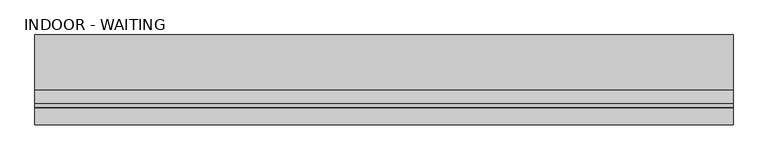
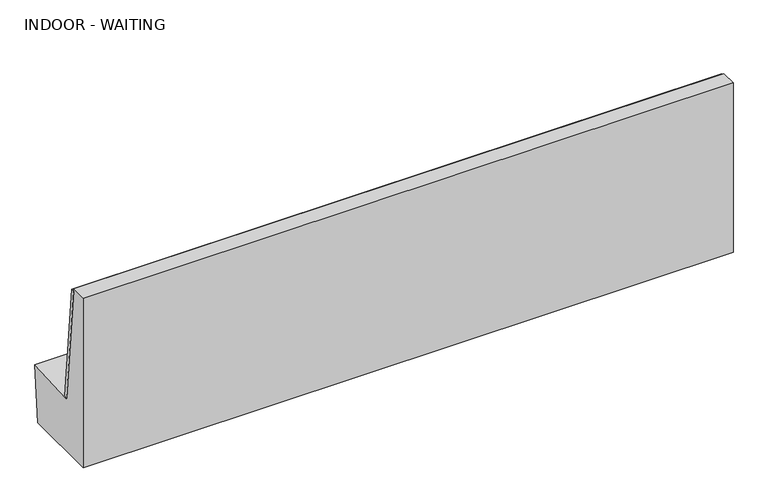
"""IFC4 building model written with IfcOpenShell, lengths in millimetres: furniture geometry, OD_CW_Booth : INDOOR - WAITING."""

import ifcopenshell
import ifcopenshell.guid

model = None  # the IFC model being written
_history = None  # IfcOwnerHistory: only IFC2X3 demands one
_inside = {}  # id of a spatial element -> (the spatial element, [elements in it])
_under = {}  # id of a project, library or spatial element -> (it, [spatial elements below it])
_declared = {}  # id of a project -> (the project, [libraries it declares])
_typed = {}  # id of a type object -> (the type object, [elements of that type])
_made_of = {}  # id of a material, layer set ... -> (it, [elements and type objects made of it])


def new_model(schema):
    """Start an empty IFC model of exactly this schema.

    Asked for "IFC4X3", IfcOpenShell would pick the latest addendum, in which some entities
    have other attributes; the version numbers below select the first issue.
    IFC2X3 requires an IfcOwnerHistory on every rooted entity: one is made here for all.
    """
    global model, _history
    if schema == "IFC4X3":
        model = ifcopenshell.file(schema_version=(4, 3, 0, 0))
    else:
        model = ifcopenshell.file(schema=schema)
    _inside.clear()
    _under.clear()
    _declared.clear()
    _typed.clear()
    _made_of.clear()
    _history = None
    if model.schema == "IFC2X3":
        org = make("IfcOrganization", Name="unknown")
        user = make(
            "IfcPersonAndOrganization",
            ThePerson=make("IfcPerson", FamilyName="unknown"),
            TheOrganization=org,
        )
        app = make(
            "IfcApplication",
            ApplicationDeveloper=org,
            Version="unknown",
            ApplicationFullName="unknown",
            ApplicationIdentifier="unknown",
        )
        _history = make(
            "IfcOwnerHistory",
            OwningUser=user,
            OwningApplication=app,
            ChangeAction="ADDED",
            CreationDate=0,
        )
    return model


def make(cls, **values):
    """One entity of the class cls with the attributes given. An attribute that is None is left unset."""
    return model.create_entity(
        cls, **{name: value for name, value in values.items() if value is not None}
    )


def rooted(cls, **values):
    """An entity with a GlobalId (a new one), such as an element, a storey or a relation."""
    return make(cls, GlobalId=ifcopenshell.guid.new(), OwnerHistory=_history, **values)


def si_unit(unit_type, name, prefix=None):
    """IfcSIUnit, for example si_unit("LENGTHUNIT", "METRE", prefix="MILLI")."""
    return make("IfcSIUnit", UnitType=unit_type, Prefix=prefix, Name=name)


def assignment(units):
    """IfcUnitAssignment: the units of a project."""
    return None if units is None else make("IfcUnitAssignment", Units=units)


def point(xyz):
    """IfcCartesianPoint."""
    return None if xyz is None else make("IfcCartesianPoint", Coordinates=xyz)


def direction(xyz):
    """IfcDirection."""
    return None if xyz is None else make("IfcDirection", DirectionRatios=xyz)


def frame(location, z_axis=None, x_axis=None):
    """IfcAxis2Placement3D, a coordinate frame: its origin and axes. An axis left out is left unset."""
    return make(
        "IfcAxis2Placement3D",
        Location=point(location),
        Axis=direction(z_axis),
        RefDirection=direction(x_axis),
    )


def origin():
    """The frame at (0, 0, 0) with its axes left unset."""
    return frame((0.0, 0.0, 0.0))


def place(relative_to, where):
    """IfcLocalPlacement: puts the frame where relative to a parent placement (None: the world)."""
    return make(
        "IfcLocalPlacement", PlacementRelTo=relative_to, RelativePlacement=where
    )


def context(
    kind, dimensions, precision=None, world=None, true_north=None, identifier=None
):
    """IfcGeometricRepresentationContext, for example the 3D "Model" context."""
    return make(
        "IfcGeometricRepresentationContext",
        ContextIdentifier=identifier,
        ContextType=kind,
        CoordinateSpaceDimension=dimensions,
        Precision=precision,
        WorldCoordinateSystem=world,
        TrueNorth=true_north,
    )


def project(units=None, contexts=None):
    """IfcProject with its units and contexts."""
    return rooted(
        "IfcProject",
        Name="project",
        RepresentationContexts=contexts,
        UnitsInContext=assignment(units),
    )


def spatial(cls, under=None, at=None, **own):
    """A site, building, storey or space (cls), placed at a placement, below another one or the project."""
    s = rooted(cls, ObjectPlacement=at, **own)
    if under is not None:
        _under.setdefault(under.id(), (under, []))[1].append(s)
    return s


def polyline(points):
    """IfcPolyline through the points."""
    return make("IfcPolyline", Points=[point(p) for p in points])


def outline(outer, holes=None, kind="AREA"):
    """IfcArbitraryClosedProfileDef: a profile drawn as a closed curve; with holes, ...WithVoids."""
    if holes is None:
        return make("IfcArbitraryClosedProfileDef", ProfileType=kind, OuterCurve=outer)
    return make(
        "IfcArbitraryProfileDefWithVoids",
        ProfileType=kind,
        OuterCurve=outer,
        InnerCurves=holes,
    )


def extrude(swept, where, along, depth):
    """IfcExtrudedAreaSolid: the profile swept, set in the frame where, extruded along a direction by depth."""
    return make(
        "IfcExtrudedAreaSolid",
        SweptArea=swept,
        Position=where,
        ExtrudedDirection=direction(along),
        Depth=depth,
    )


def shape(context_of_items, identifier, shape_type, items):
    """IfcShapeRepresentation: the items that make up one representation, for example the "Body"."""
    return make(
        "IfcShapeRepresentation",
        ContextOfItems=context_of_items,
        RepresentationIdentifier=identifier,
        RepresentationType=shape_type,
        Items=items,
    )


def source(mapping_origin, context_of_items, identifier, shape_type, items):
    """IfcRepresentationMap: a shape defined once, which mapped items show again and again."""
    return make(
        "IfcRepresentationMap",
        MappingOrigin=mapping_origin,
        MappedRepresentation=shape(context_of_items, identifier, shape_type, items),
    )


def transform(
    local_origin,
    x_axis=None,
    y_axis=None,
    z_axis=None,
    scale=None,
    scale2=None,
    scale3=None,
    uniform=True,
):
    """IfcCartesianTransformationOperator3D, or its non-uniform kind. x_axis, y_axis, z_axis: its Axis1, 2, 3."""
    if uniform:
        return make(
            "IfcCartesianTransformationOperator3D",
            Axis1=direction(x_axis),
            Axis2=direction(y_axis),
            LocalOrigin=point(local_origin),
            Scale=scale,
            Axis3=direction(z_axis),
        )
    return make(
        "IfcCartesianTransformationOperator3DnonUniform",
        Axis1=direction(x_axis),
        Axis2=direction(y_axis),
        LocalOrigin=point(local_origin),
        Scale=scale,
        Axis3=direction(z_axis),
        Scale2=scale2,
        Scale3=scale3,
    )


def mapped(mapping_source, mapping_target):
    """IfcMappedItem: shows the shape of a source again, moved by a transform."""
    return make(
        "IfcMappedItem", MappingSource=mapping_source, MappingTarget=mapping_target
    )


def made_of(thing, what):
    """Note that an element or type object is made of a material, layer set ...; save() writes the relation."""
    if what is not None:
        _made_of.setdefault(what.id(), (what, []))[1].append(thing)
    return thing


def element(
    cls,
    number,
    at=None,
    inside=None,
    cuts=None,
    type_object=None,
    material=None,
    context=None,
    identifier="Body",
    shape_type=None,
    held_by="IfcProductDefinitionShape",
    body=None,
    shapes=None,
    **own,
):
    """One element of the class cls, such as IfcWall. Its Tag is "e" and its number.

    at: its placement. inside: the storey or other place that contains it. cuts: it is an
    opening in that element (IfcRelVoidsElement). A single representation is given by context,
    identifier, shape_type and body (its items); several are given by shapes. held_by: the class
    of the entity that holds the representations. save() writes the other relations.
    """
    e = rooted(cls, Tag="e%d" % number, ObjectPlacement=at, **own)
    if body is not None:
        shapes = [shape(context, identifier, shape_type, body)]
    if shapes is not None:
        e.Representation = make(held_by, Representations=shapes)
    if inside is not None:
        _inside.setdefault(inside.id(), (inside, []))[1].append(e)
    if cuts is not None:
        rooted(
            "IfcRelVoidsElement", RelatingBuildingElement=cuts, RelatedOpeningElement=e
        )
    if type_object is not None:
        _typed.setdefault(type_object.id(), (type_object, []))[1].append(e)
    return made_of(e, material)


def aggregate(whole, parts):
    """IfcRelAggregates: a whole, such as a stair, and the parts it consists of."""
    return rooted("IfcRelAggregates", RelatingObject=whole, RelatedObjects=parts)


def save(model, path):
    """Write the relations noted so far, then the file.

    IfcRelAggregates (storeys below a building ...), IfcRelContainedInSpatialStructure (elements
    in a storey), IfcRelDefinesByType, IfcRelAssociatesMaterial and IfcRelDeclares: one each for
    every whole, place, type object, material and project.
    """
    for whole, parts in _under.values():
        aggregate(whole, parts)
    for where, things in _inside.values():
        rooted(
            "IfcRelContainedInSpatialStructure",
            RelatedElements=things,
            RelatingStructure=where,
        )
    for kind, things in _typed.values():
        rooted("IfcRelDefinesByType", RelatedObjects=things, RelatingType=kind)
    for what, things in _made_of.values():
        rooted("IfcRelAssociatesMaterial", RelatedObjects=things, RelatingMaterial=what)
    for by, libraries in _declared.values():
        rooted("IfcRelDeclares", RelatingContext=by, RelatedDefinitions=libraries)
    model.write(path)


def indoor_waiting_8bc71f9b(model_context):
    return source(origin(), model_context, "Body", "SweptSolid", [
        extrude(outline(polyline([(0.0, -5064.5281442), (0.0, 0.0), (25.4, 0.0), (25.4, -5064.5281442), (0.0, -5064.5281442)])), frame((5083.2658491, -358.2049359, 438.8309433), z_axis=(0.0, -0.10452846326765197, 0.9945218953682735), x_axis=(0.0, -0.9945218953682735, -0.10452846326765197)), (0.0, 0.0, 1.0), 944.7333479),
        extrude(outline(polyline([(-609.6, 1397.0), (-484.4524721, 1397.0), (-382.9385128, 431.1591941), (43.0849153, 453.4861359), (3.4100193, 0.0), (-609.6, 0.0), (-609.6, 1397.0)])), frame((18.7377049, 0.0, 0.0), z_axis=(1.0, 0.0, 0.0), x_axis=(0.0, 1.0, 0.0)), (0.0, 0.0, 1.0), 5064.5281442),
    ])


if __name__ == "__main__":
    model = new_model("IFC4")
    model_context = context("Model", 3, world=origin())
    ifc_project = project(units=[si_unit("LENGTHUNIT", "METRE", prefix="MILLI")], contexts=[model_context])
    site = spatial("IfcSite", under=ifc_project)
    building = spatial("IfcBuilding", under=site)
    placement = place(None, origin())
    indoor_waiting_shape = indoor_waiting_8bc71f9b(model_context)
    element("IfcFurniture", 1, ObjectType="OD_CW_Booth : INDOOR - WAITING", at=placement, inside=building, context=model_context, shape_type="MappedRepresentation", body=[
        mapped(indoor_waiting_shape, transform((0.0, 0.0, 0.0), x_axis=(1.0, 0.0, 0.0), y_axis=(0.0, 1.0, 0.0), z_axis=(0.0, 0.0, 1.0))),
    ])
    save(model, "model.ifc")

# Revit data of these elements
# Type "OD_CW_Booth : INDOOR - WAITING"
#   Width = 4' - 0"
#   OD_CW_Width [instance default] = 2' - 10"
#   OD_CW_Length [instance default] = 26' - 1 83/256"
#   OD_CW_Height [instance default] = 2' - 3"
#   Height = 3' - 0"
#   Depth = 2' - 0"
#   Seating Count [instance default] = 10
#   back = Casework-oakfire
#   OD_CW_Material_Front Panel [instance default] = none
#   OD_CW_Material_Body [instance default] = none
# Element 1 (IfcFurniture, "OD_CW_Booth : INDOOR - WAITING")
#   OD_CW_Length = 16' - 7.39087"
#   Seating Count = 6
#   OD_CW_Material_Body = WOOD-OAKFIRE
#   Materials on its faces: "WOOD-OAKFIRE", "Casework-oakfire"
# Materials
#   "Casework-oakfire": class "Miscellaneous", colour RGB 164 164 164, transparency 0, Cost = 0
#   "WOOD-OAKFIRE": class "Wood", colour RGB 198 202 183, transparency 0, Description = "Generic wood", Cost = 0
